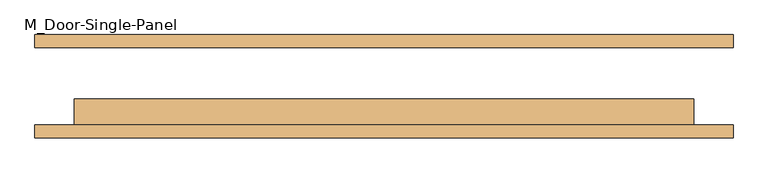
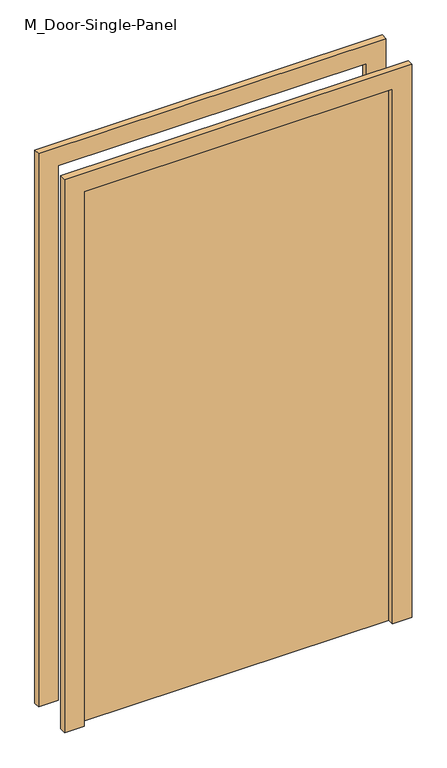
"""IFC4 building model written with IfcOpenShell, lengths in millimetres: door geometry, M_Door-Single-Panel : 1200 x 2200mm DAPC."""

from ifc_helpers import new_model, si_unit, frame, origin, origin_with_axes, place, context, project, spatial, polyline, outline, extrude, source, transform, mapped, element, save


def m_door_single_panel_314eda02(model_context):
    return source(origin(), model_context, "Body", "SweptSolid", [
        extrude(outline(polyline([(600.0, -25.0), (600.0, -75.0), (-600.0, -75.0), (-600.0, -25.0), (600.0, -25.0)])), origin_with_axes(), (0.0, 0.0, 1.0), 2200.0),
        extrude(outline(polyline([(2276.2, 676.2), (2276.2, -676.2), (0.0, -676.2), (0.0, -600.0), (2200.0, -600.0), (2200.0, 600.0), (0.0, 600.0), (0.0, 676.2), (2276.2, 676.2)])), frame((0.0, 75.0, 0.0), z_axis=(0.0, 1.0, 0.0), x_axis=(0.0, 0.0, 1.0)), (0.0, 0.0, 1.0), 25.0),
        extrude(outline(polyline([(2276.2, -676.2), (0.0, -676.2), (0.0, -600.0), (2200.0, -600.0), (2200.0, 600.0), (0.0, 600.0), (0.0, 676.2), (2276.2, 676.2), (2276.2, -676.2)])), frame((0.0, -100.0, 0.0), z_axis=(0.0, 1.0, 0.0), x_axis=(0.0, 0.0, 1.0)), (0.0, 0.0, 1.0), 25.0),
    ])


if __name__ == "__main__":
    model = new_model("IFC4")
    model_context = context("Model", 3, world=origin())
    ifc_project = project(units=[si_unit("LENGTHUNIT", "METRE", prefix="MILLI")], contexts=[model_context])
    site = spatial("IfcSite", under=ifc_project)
    building = spatial("IfcBuilding", under=site)
    placement = place(None, origin())
    m_door_single_panel_shape = m_door_single_panel_314eda02(model_context)
    element("IfcDoor", 1, ObjectType="M_Door-Single-Panel : 1200 x 2200mm DAPC", at=placement, inside=building, context=model_context, shape_type="MappedRepresentation", body=[
        mapped(m_door_single_panel_shape, transform((0.0, 0.0, 0.0), x_axis=(1.0, 0.0, 0.0), y_axis=(0.0, 1.0, 0.0), z_axis=(0.0, 0.0, 1.0))),
    ])
    save(model, "model.ifc")

# Revit data of these elements
# Type "M_Door-Single-Panel : 1200 x 2200mm DAPC"
#   Type Mark = "49"
#   Construction Type Id = "DOOR"
#   Analytic Construction = "Wooden"
#   Thickness = 0.05 m
#   Thermal Resistance (R) = 0.455703 (m²·K)/W
#   Swing Angle [instance default] = 90.00°
#   Heat Transfer Coefficient (U) = 2.19465 W/(m²·K)
#   Height = 2.20 m
#   Trim Projection Ext = 0.025 m
#   Trim Projection Int = 0.025 m
#   Trim Width = 0.08 m
#   Width = 1.20 m
#   Define Thermal Properties by = 1
#   Panel Material = Wood - Birch - Solid Stained Light Low Gloss
#   Trim Material = Paint - Sienna
#   Visual Light Transmittance = 0
#   Solar Heat Gain Coefficient = 0
#   Function = (empty or 0)
#   Wall Closure = (empty or 0)
# Element 1 (IfcDoor, "M_Door-Single-Panel : 1200 x 2200mm DAPC")
#   Materials on its faces: "Paint - Sienna", "Wood - Birch - Solid Stained Light Low Gloss"
# Materials
#   "Wood - Birch - Solid Stained Light Low Gloss": class "Wood", colour RGB 210 159 95, transparency 0, Cost = 0
#   "Paint - Sienna": class "Miscellaneous", colour RGB 118 70 51, transparency 0, Cost = 0
